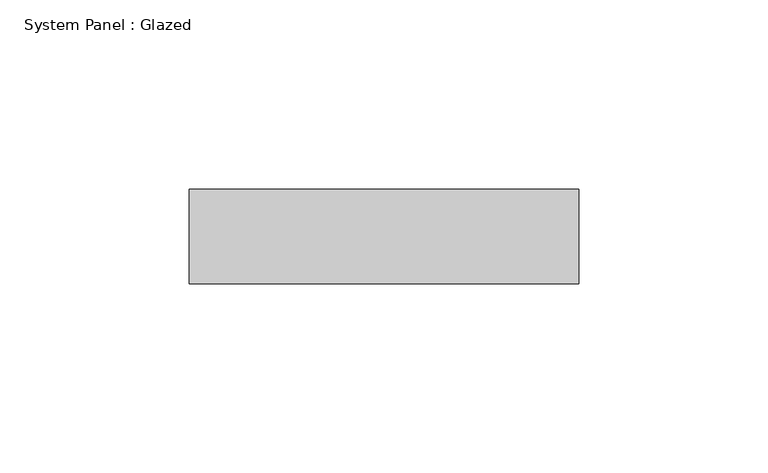
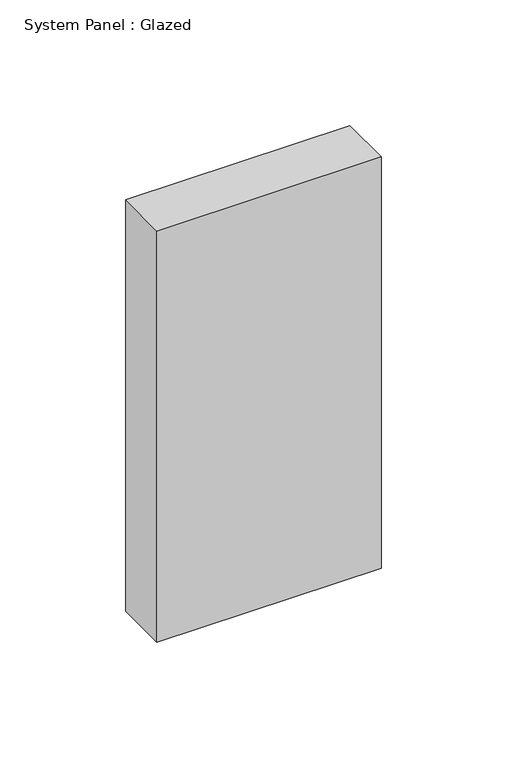
"""IFC4 building model written with IfcOpenShell, lengths in millimetres: plate geometry, System Panel : Glazed."""

from ifc_helpers import new_model, si_unit, origin, origin_with_axes, place, context, project, spatial, polyline, outline, extrude, source, transform, mapped, element, save


def system_panel_glazed_4b393385(model_context):
    return source(origin(), model_context, "Body", "SweptSolid", [
        extrude(outline(polyline([(51.5698685, 24.5), (-51.5698685, 24.5), (-51.5698685, 49.5), (51.5698685, 49.5), (51.5698685, 24.5)])), origin_with_axes(), (0.0, 0.0, 1.0), 200.0),
    ])


if __name__ == "__main__":
    model = new_model("IFC4")
    model_context = context("Model", 3, world=origin())
    ifc_project = project(units=[si_unit("LENGTHUNIT", "METRE", prefix="MILLI")], contexts=[model_context])
    site = spatial("IfcSite", under=ifc_project)
    building = spatial("IfcBuilding", under=site)
    placement = place(None, origin())
    system_panel_glazed_shape = system_panel_glazed_4b393385(model_context)
    element("IfcPlate", 1, ObjectType="System Panel : Glazed", at=placement, inside=building, context=model_context, shape_type="MappedRepresentation", body=[
        mapped(system_panel_glazed_shape, transform((0.0, 0.0, 0.0), x_axis=(1.0, 0.0, 0.0), y_axis=(0.0, 1.0, 0.0), z_axis=(0.0, 0.0, 1.0))),
    ])
    save(model, "model.ifc")

# Revit data of these elements
# Element 1 (IfcPlate, "System Panel : Glazed")
#   Materials on its faces: "Glass"
# Materials
#   "Glass": class "Glass", colour RGB 218 227 224, transparency 0.85, Description = "Soda Lime Glass", Cost = 0
